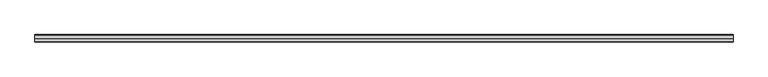
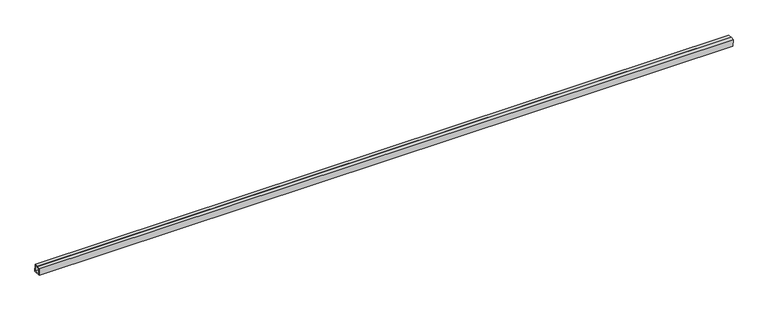
"""IFC4 building model written with IfcOpenShell, lengths in millimetres: proxy geometry, Inner panel:Inner panel:1:Inner panel:1 : Inner panel:Inner panel:300324:2:Inner panel:1:Inner panel:1 : Inner panel:Inner panel:300324:2 : Inner panel:Inner panel:1:Inner panel:1 : Inner panel:Inner panel:300324:300043:1 : Inner panel:Inner panel:1:Inner panel:1 : Inner panel:Inner panel:300324:2:Inner panel:1:Inner panel:1 : Inner panel:Inner panel:300324:2 : Inner panel:Inner panel:1:Inner panel:1 : Inner panel:Inner panel:300324:300043:308120."""

from ifc_helpers import new_model, si_unit, frame, origin, place, context, project, spatial, polyline, outline, extrude, source, transform, mapped, element, save


def generic_models_b7bf941d(model_context):
    return source(origin(), model_context, "Body", "SweptSolid", [
        extrude(outline(polyline([(-580608.3153149, 3882.914021), (-580590.0748917, 3883.6740386), (-580588.488768, 3845.6070685), (-580626.5557381, 3844.0209448), (-580628.1418618, 3882.0879149), (-580609.9014386, 3882.8479325), (-580609.8023059, 3880.4687469), (-580625.6635434, 3879.807862), (-580624.2756852, 3846.4992631), (-580590.9670863, 3847.8871214), (-580592.3549446, 3881.1957202), (-580608.2161822, 3880.5348354), (-580608.3153149, 3882.914021)])), frame((593141.1867239, 0.0, 0.0), z_axis=(1.0, 0.0, 0.0), x_axis=(0.0, 1.0, 0.0)), (0.0, 0.0, 1.0), 3657.6),
    ])


if __name__ == "__main__":
    model = new_model("IFC4")
    model_context = context("Model", 3, world=origin())
    ifc_project = project(units=[si_unit("LENGTHUNIT", "METRE", prefix="MILLI")], contexts=[model_context])
    site = spatial("IfcSite", under=ifc_project)
    building = spatial("IfcBuilding", under=site)
    placement = place(None, origin())
    generic_models_shape = generic_models_b7bf941d(model_context)
    element("IfcBuildingElementProxy", 1, Name="Inner panel:Inner panel:1:Inner panel:1 : Inner panel:Inner panel:300324:2:Inner panel:1:Inner panel:1 : Inner panel:Inner panel:300324:2 : Inner panel:Inner panel:1:Inner panel:1 : Inner panel:Inner panel:300324:300043:1 : Inner panel:Inner panel:1:Inner panel:1 : Inner panel:Inner panel:300324:2:Inner panel:1:Inner panel:1 : Inner panel:Inner panel:300324:2 : Inner panel:Inner panel:1:Inner panel:1 : Inner panel:Inner panel:300324:300043:308120", ObjectType="Inner panel:Inner panel:1:Inner panel:1 : Inner panel:Inner panel:300324:2:Inner panel:1:Inner panel:1 : Inner panel:Inner panel:300324:2 : Inner panel:Inner panel:1:Inner panel:1 : Inner panel:Inner panel:300324:300043:1 : Inner panel:Inner panel:1:Inner panel:1 : Inner panel:Inner panel:300324:2:Inner panel:1:Inner panel:1 : Inner panel:Inner panel:300324:2 : Inner panel:Inner panel:1:Inner panel:1 : Inner panel:Inner panel:300324:300043:308120", at=placement, inside=building, context=model_context, shape_type="MappedRepresentation", body=[
        mapped(generic_models_shape, transform((0.0, 0.0, 0.0), x_axis=(1.0, 0.0, 0.0), y_axis=(0.0, 1.0, 0.0), z_axis=(0.0, 0.0, 1.0))),
    ])
    save(model, "model.ifc")

# Revit data of these elements
# Type "Inner panel:Inner panel:1:Inner panel:1 : Inner panel:Inner panel:300324:2:Inner panel:1:Inner panel:1 : Inner panel:Inner panel:300324:2 : Inner panel:Inner panel:1:Inner panel:1 : Inner panel:Inner panel:300324:300043:1 : Inner panel:Inner panel:1:Inner panel:1 : Inner panel:Inner panel:300324:2:Inner panel:1:Inner panel:1 : Inner panel:Inner panel:300324:2 : Inner panel:Inner panel:1:Inner panel:1 : Inner panel:Inner panel:300324:300043:308120"
#   NameOverride = "Inner panel:Inner panel:1:Inner panel:1 : Inner panel:Inner panel:300324:2:Inner panel:1:Inner panel:1 : Inner panel:Inner panel:300324:2 : Inner panel:Inner panel:1:Inner panel:1 : Inner panel:Inner panel:300324:300043:308120"
#   ObjectTypeOverride = "Inner panel:1:Inner panel:1 : Inner panel:Inner panel:300324:2 : Inner panel:Inner panel:1:Inner panel:1 : Inner panel:Inner panel:300324:300043"
#   Reference = "Inner panel"
#   Tag = "308120"
# Element 1 (IfcBuildingElementProxy, "Inner panel:Inner panel:1:Inner panel:1 : Inner panel:Inner panel:300324:2:Inner panel:1:Inner panel:1 : Inner panel:Inner panel:300324:2 : Inner panel:Inner panel:1:Inner panel:1 : Inner panel:Inner panel:300324:300043:1 : Inner panel:Inner panel:1:Inner panel:1 : Inner panel:Inner panel:300324:2:Inner panel:1:Inner panel:1 : Inner panel:Inner panel:300324:2 : Inner panel:Inner panel:1:Inner panel:1 : Inner panel:Inner panel:300324:300043:308120")
#   Materials on its faces: "1 1/2\" X 1 1/2\" SPLIT-SEAM SQUARE TUBING (~24\" CANTILEVER FROM C.L. OF GLULAM)"
# Materials
#   "1 1/2\" X 1 1/2\" SPLIT-SEAM SQUARE TUBING (~24\" CANTILEVER FROM C.L. OF GLULAM)": class "Unassigned", colour RGB 202 201 200, transparency 0, Cost = 0
